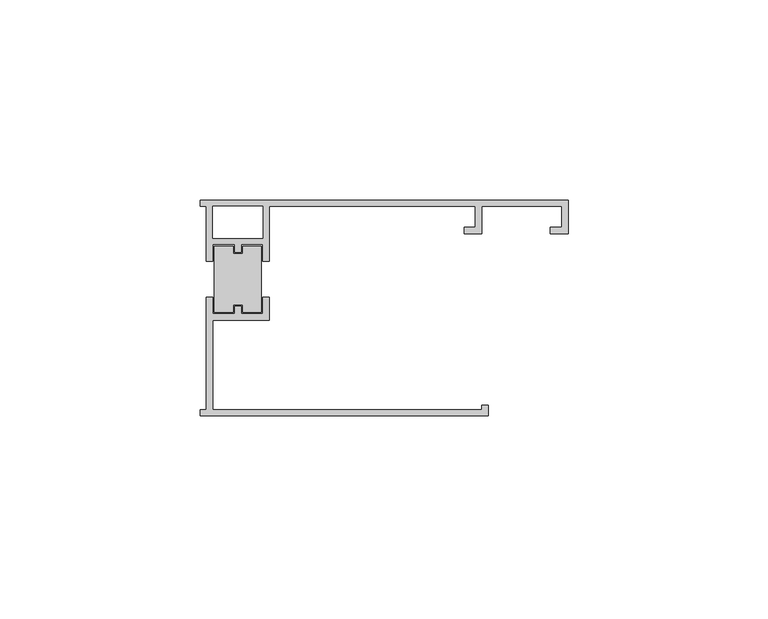
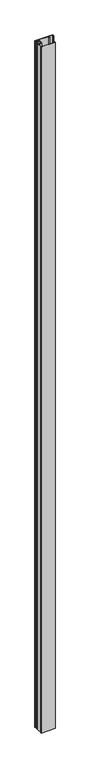
"""IFC4 building model written with IfcOpenShell, lengths in millimetres: proxy geometry, Generic Models 2:Generic Models 2:310765:Generic Models 2:310765 : Generic Models 2:Generic Models 2:310765:10 : Generic Models 2:Generic Models 2:310765:Generic Models 2:310765 : Generic Models 2:Generic Models 2:310765:300385."""

from ifc_helpers import new_model, si_unit, frame, origin, place, context, project, spatial, polyline, outline, extrude, source, transform, mapped, element, save


def generic_models_736596d6(model_context):
    return source(origin(), model_context, "Body", "SweptSolid", [
        extrude(outline(polyline([(582723.4848462, -579060.466762), (582718.7873476, -579060.466762), (582718.7873476, -579058.5413465), (582716.4060976, -579058.5413465), (582716.4060976, -579060.466762), (582711.7085989, -579060.466762), (582711.7085989, -579043.9145058), (582716.4060976, -579043.9145058), (582716.4060976, -579045.8399212), (582718.7873476, -579045.8399212), (582718.7873476, -579043.9145058), (582723.4848462, -579043.9145058), (582723.4848462, -579060.466762)])), frame((0.0, 0.0, 6.2703961), z_axis=(0.0, 0.0, 1.0), x_axis=(1.0, 0.0, 0.0)), (0.0, 0.0, 1.0), 3695.7),
        extrude(outline(polyline([(582800.1367239, -579040.8458673), (582795.7493974, -579040.8458673), (582795.7493974, -579039.2583673), (582798.5492239, -579039.2583673), (582798.5492239, -579033.9869958), (582778.5492239, -579033.9869958), (582778.5492239, -579040.8458673), (582774.1618974, -579040.8458673), (582774.1618974, -579039.2583673), (582776.9617239, -579039.2583673), (582776.9617239, -579033.9869958), (582725.4692212, -579033.9869958), (582725.4692212, -579047.6848183), (582723.8817212, -579047.6848183), (582723.8817212, -579043.5176308), (582718.3904726, -579043.5176308), (582718.3904726, -579045.4430462), (582716.8029726, -579045.4430462), (582716.8029726, -579043.5176308), (582711.3117239, -579043.5176308), (582711.3117239, -579047.6848183), (582709.7242239, -579047.6848183), (582709.7242239, -579033.9869958), (582708.1367239, -579033.9869958), (582708.1367239, -579032.3994958), (582800.1367239, -579032.3994958), (582800.1367239, -579040.8458673)]), holes=[polyline([(582723.8817212, -579033.9869958), (582711.3117239, -579033.9869958), (582711.3117239, -579041.9301308), (582723.8817212, -579041.9301308), (582723.8817212, -579033.9869958)])]), frame((0.0, 0.0, 6.2703961), z_axis=(0.0, 0.0, 1.0), x_axis=(1.0, 0.0, 0.0)), (0.0, 0.0, 1.0), 3695.7),
        extrude(outline(polyline([(582708.1367239, -579084.8119958), (582709.7242239, -579084.8119958), (582709.7242239, -579056.6964495), (582711.3117239, -579056.6964495), (582711.3117239, -579060.863637), (582716.8029726, -579060.863637), (582716.8029726, -579058.9382215), (582718.3904726, -579058.9382215), (582718.3904726, -579060.863637), (582723.8817212, -579060.863637), (582723.8817212, -579056.6964495), (582725.4692212, -579056.6964495), (582725.4692212, -579062.451137), (582711.3117239, -579062.451137), (582711.3117239, -579084.8119958), (582778.5492239, -579084.8119958), (582778.5492239, -579083.6844059), (582780.1367239, -579083.6844059), (582780.1367239, -579086.3994958), (582708.1367239, -579086.3994958), (582708.1367239, -579084.8119958)])), frame((0.0, 0.0, 6.2703961), z_axis=(0.0, 0.0, 1.0), x_axis=(1.0, 0.0, 0.0)), (0.0, 0.0, 1.0), 3695.7),
    ])


if __name__ == "__main__":
    model = new_model("IFC4")
    model_context = context("Model", 3, world=origin())
    ifc_project = project(units=[si_unit("LENGTHUNIT", "METRE", prefix="MILLI")], contexts=[model_context])
    site = spatial("IfcSite", under=ifc_project)
    building = spatial("IfcBuilding", under=site)
    placement = place(None, origin())
    generic_models_shape = generic_models_736596d6(model_context)
    element("IfcBuildingElementProxy", 1, Name="Generic Models 2:Generic Models 2:310765:Generic Models 2:310765 : Generic Models 2:Generic Models 2:310765:10 : Generic Models 2:Generic Models 2:310765:Generic Models 2:310765 : Generic Models 2:Generic Models 2:310765:300385", ObjectType="Generic Models 2:Generic Models 2:310765:Generic Models 2:310765 : Generic Models 2:Generic Models 2:310765:10 : Generic Models 2:Generic Models 2:310765:Generic Models 2:310765 : Generic Models 2:Generic Models 2:310765:300385", at=placement, inside=building, context=model_context, shape_type="MappedRepresentation", body=[
        mapped(generic_models_shape, transform((0.0, 0.0, 0.0), x_axis=(1.0, 0.0, 0.0), y_axis=(0.0, 1.0, 0.0), z_axis=(0.0, 0.0, 1.0))),
    ])
    save(model, "model.ifc")

# Revit data of these elements
# Type "Generic Models 2:Generic Models 2:310765:Generic Models 2:310765 : Generic Models 2:Generic Models 2:310765:10 : Generic Models 2:Generic Models 2:310765:Generic Models 2:310765 : Generic Models 2:Generic Models 2:310765:300385"
#   NameOverride = "Generic Models 2:Generic Models 2:310765:Generic Models 2:310765 : Generic Models 2:Generic Models 2:310765:300385"
#   ObjectTypeOverride = "Generic Models 2:310765 : Generic Models 2:Generic Models 2:310765"
#   Reference = "Generic Models 2"
#   Tag = "300385"
# Element 1 (IfcBuildingElementProxy, "Generic Models 2:Generic Models 2:310765:Generic Models 2:310765 : Generic Models 2:Generic Models 2:310765:10 : Generic Models 2:Generic Models 2:310765:Generic Models 2:310765 : Generic Models 2:Generic Models 2:310765:300385")
#   Materials on its faces: "THERMAL BROKEN ALUMINUM STOREFRONT FOR POLYCARBONATE"
# Materials
#   "THERMAL BROKEN ALUMINUM STOREFRONT FOR POLYCARBONATE": class "Unassigned", colour RGB 244 244 244, transparency 0, Keynote = "M07611300.01", Cost = 0
